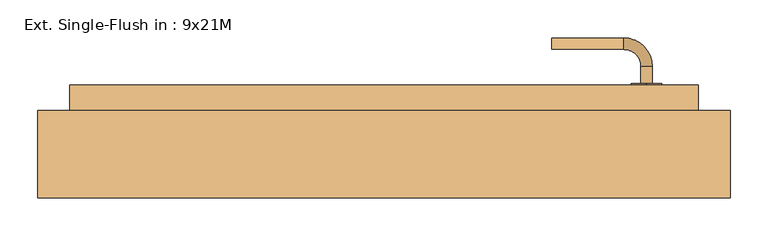
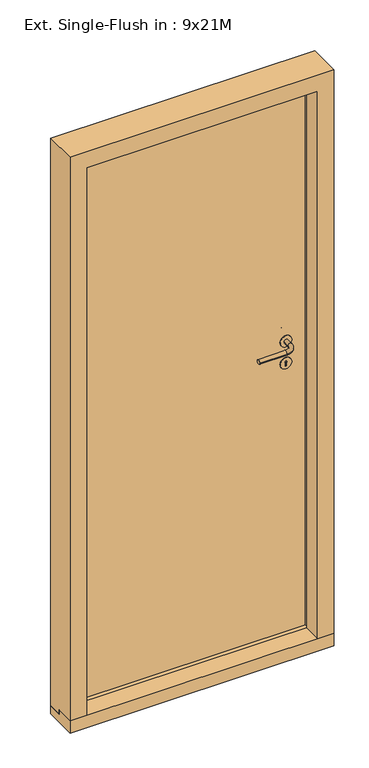
"""IFC4 building model written with IfcOpenShell, lengths in millimetres: door geometry, Ext. Single-Flush in : 9x21M."""

import ifcopenshell
import ifcopenshell.guid

model = None  # the IFC model being written
_history = None  # IfcOwnerHistory: only IFC2X3 demands one
_inside = {}  # id of a spatial element -> (the spatial element, [elements in it])
_under = {}  # id of a project, library or spatial element -> (it, [spatial elements below it])
_declared = {}  # id of a project -> (the project, [libraries it declares])
_typed = {}  # id of a type object -> (the type object, [elements of that type])
_made_of = {}  # id of a material, layer set ... -> (it, [elements and type objects made of it])


def new_model(schema):
    """Start an empty IFC model of exactly this schema.

    Asked for "IFC4X3", IfcOpenShell would pick the latest addendum, in which some entities
    have other attributes; the version numbers below select the first issue.
    IFC2X3 requires an IfcOwnerHistory on every rooted entity: one is made here for all.
    """
    global model, _history
    if schema == "IFC4X3":
        model = ifcopenshell.file(schema_version=(4, 3, 0, 0))
    else:
        model = ifcopenshell.file(schema=schema)
    _inside.clear()
    _under.clear()
    _declared.clear()
    _typed.clear()
    _made_of.clear()
    _history = None
    if model.schema == "IFC2X3":
        org = make("IfcOrganization", Name="unknown")
        user = make(
            "IfcPersonAndOrganization",
            ThePerson=make("IfcPerson", FamilyName="unknown"),
            TheOrganization=org,
        )
        app = make(
            "IfcApplication",
            ApplicationDeveloper=org,
            Version="unknown",
            ApplicationFullName="unknown",
            ApplicationIdentifier="unknown",
        )
        _history = make(
            "IfcOwnerHistory",
            OwningUser=user,
            OwningApplication=app,
            ChangeAction="ADDED",
            CreationDate=0,
        )
    return model


def make(cls, **values):
    """One entity of the class cls with the attributes given. An attribute that is None is left unset."""
    return model.create_entity(
        cls, **{name: value for name, value in values.items() if value is not None}
    )


def rooted(cls, **values):
    """An entity with a GlobalId (a new one), such as an element, a storey or a relation."""
    return make(cls, GlobalId=ifcopenshell.guid.new(), OwnerHistory=_history, **values)


def si_unit(unit_type, name, prefix=None):
    """IfcSIUnit, for example si_unit("LENGTHUNIT", "METRE", prefix="MILLI")."""
    return make("IfcSIUnit", UnitType=unit_type, Prefix=prefix, Name=name)


def assignment(units):
    """IfcUnitAssignment: the units of a project."""
    return None if units is None else make("IfcUnitAssignment", Units=units)


def point(xyz):
    """IfcCartesianPoint."""
    return None if xyz is None else make("IfcCartesianPoint", Coordinates=xyz)


def direction(xyz):
    """IfcDirection."""
    return None if xyz is None else make("IfcDirection", DirectionRatios=xyz)


def frame(location, z_axis=None, x_axis=None):
    """IfcAxis2Placement3D, a coordinate frame: its origin and axes. An axis left out is left unset."""
    return make(
        "IfcAxis2Placement3D",
        Location=point(location),
        Axis=direction(z_axis),
        RefDirection=direction(x_axis),
    )


def frame_2d(location, x_axis=None):
    """IfcAxis2Placement2D, a coordinate frame in the plane: its origin and x axis."""
    return make(
        "IfcAxis2Placement2D", Location=point(location), RefDirection=direction(x_axis)
    )


def origin():
    """The frame at (0, 0, 0) with its axes left unset."""
    return frame((0.0, 0.0, 0.0))


def place(relative_to, where):
    """IfcLocalPlacement: puts the frame where relative to a parent placement (None: the world)."""
    return make(
        "IfcLocalPlacement", PlacementRelTo=relative_to, RelativePlacement=where
    )


def context(
    kind, dimensions, precision=None, world=None, true_north=None, identifier=None
):
    """IfcGeometricRepresentationContext, for example the 3D "Model" context."""
    return make(
        "IfcGeometricRepresentationContext",
        ContextIdentifier=identifier,
        ContextType=kind,
        CoordinateSpaceDimension=dimensions,
        Precision=precision,
        WorldCoordinateSystem=world,
        TrueNorth=true_north,
    )


def project(units=None, contexts=None):
    """IfcProject with its units and contexts."""
    return rooted(
        "IfcProject",
        Name="project",
        RepresentationContexts=contexts,
        UnitsInContext=assignment(units),
    )


def spatial(cls, under=None, at=None, **own):
    """A site, building, storey or space (cls), placed at a placement, below another one or the project."""
    s = rooted(cls, ObjectPlacement=at, **own)
    if under is not None:
        _under.setdefault(under.id(), (under, []))[1].append(s)
    return s


def polyline(points):
    """IfcPolyline through the points."""
    return make("IfcPolyline", Points=[point(p) for p in points])


def circle_curve(where, radius):
    """IfcCircle in the frame where."""
    return make("IfcCircle", Position=where, Radius=radius)


def ellipse_curve(where, semi_axis1, semi_axis2):
    """IfcEllipse in the frame where."""
    return make(
        "IfcEllipse", Position=where, SemiAxis1=semi_axis1, SemiAxis2=semi_axis2
    )


def trimmed(basis, trim1, trim2, sense, master):
    """IfcTrimmedCurve: the piece of a basis curve between two trims."""
    return make(
        "IfcTrimmedCurve",
        BasisCurve=basis,
        Trim1=trim1,
        Trim2=trim2,
        SenseAgreement=sense,
        MasterRepresentation=master,
    )


def segment(curve, same_sense, transition):
    """IfcCompositeCurveSegment."""
    return make(
        "IfcCompositeCurveSegment",
        Transition=transition,
        SameSense=same_sense,
        ParentCurve=curve,
    )


def composite_curve(segments, self_intersect=None):
    """IfcCompositeCurve: segments joined end to end."""
    return make("IfcCompositeCurve", Segments=segments, SelfIntersect=self_intersect)


def outline(outer, holes=None, kind="AREA"):
    """IfcArbitraryClosedProfileDef: a profile drawn as a closed curve; with holes, ...WithVoids."""
    if holes is None:
        return make("IfcArbitraryClosedProfileDef", ProfileType=kind, OuterCurve=outer)
    return make(
        "IfcArbitraryProfileDefWithVoids",
        ProfileType=kind,
        OuterCurve=outer,
        InnerCurves=holes,
    )


def extrude(swept, where, along, depth):
    """IfcExtrudedAreaSolid: the profile swept, set in the frame where, extruded along a direction by depth."""
    return make(
        "IfcExtrudedAreaSolid",
        SweptArea=swept,
        Position=where,
        ExtrudedDirection=direction(along),
        Depth=depth,
    )


def faces_of(points, faces, orient=None, outer=None):
    """IfcFace entities. A face is a list of loops; a loop is a list of indices into points, from 0.

    orient and outer hold one flag for each loop. By default every Orientation is true, the
    first loop of a face is its IfcFaceOuterBound and the others are IfcFaceBound.
    """
    made = []
    for i, loops in enumerate(faces):
        bounds = []
        for j, loop in enumerate(loops):
            is_outer = j == 0 if outer is None else outer[i][j]
            bounds.append(
                make(
                    "IfcFaceOuterBound" if is_outer else "IfcFaceBound",
                    Bound=make("IfcPolyLoop", Polygon=[points[k] for k in loop]),
                    Orientation=True if orient is None else orient[i][j],
                )
            )
        made.append(make("IfcFace", Bounds=bounds))
    return made


def faceted_brep(points, faces, orient=None, outer=None, voids=None):
    """IfcFacetedBrep: a solid bounded by flat faces; with voids (closed shells), ...WithVoids."""
    shared = [point(p) for p in points]
    hull = make("IfcClosedShell", CfsFaces=faces_of(shared, faces, orient, outer))
    if voids is None:
        return make("IfcFacetedBrep", Outer=hull)
    return make(
        "IfcFacetedBrepWithVoids",
        Outer=hull,
        Voids=[
            make(cls, CfsFaces=faces_of(shared, fs, o, b)) for cls, fs, o, b in voids
        ],
    )


def shape(context_of_items, identifier, shape_type, items):
    """IfcShapeRepresentation: the items that make up one representation, for example the "Body"."""
    return make(
        "IfcShapeRepresentation",
        ContextOfItems=context_of_items,
        RepresentationIdentifier=identifier,
        RepresentationType=shape_type,
        Items=items,
    )


def source(mapping_origin, context_of_items, identifier, shape_type, items):
    """IfcRepresentationMap: a shape defined once, which mapped items show again and again."""
    return make(
        "IfcRepresentationMap",
        MappingOrigin=mapping_origin,
        MappedRepresentation=shape(context_of_items, identifier, shape_type, items),
    )


def transform(
    local_origin,
    x_axis=None,
    y_axis=None,
    z_axis=None,
    scale=None,
    scale2=None,
    scale3=None,
    uniform=True,
):
    """IfcCartesianTransformationOperator3D, or its non-uniform kind. x_axis, y_axis, z_axis: its Axis1, 2, 3."""
    if uniform:
        return make(
            "IfcCartesianTransformationOperator3D",
            Axis1=direction(x_axis),
            Axis2=direction(y_axis),
            LocalOrigin=point(local_origin),
            Scale=scale,
            Axis3=direction(z_axis),
        )
    return make(
        "IfcCartesianTransformationOperator3DnonUniform",
        Axis1=direction(x_axis),
        Axis2=direction(y_axis),
        LocalOrigin=point(local_origin),
        Scale=scale,
        Axis3=direction(z_axis),
        Scale2=scale2,
        Scale3=scale3,
    )


def mapped(mapping_source, mapping_target):
    """IfcMappedItem: shows the shape of a source again, moved by a transform."""
    return make(
        "IfcMappedItem", MappingSource=mapping_source, MappingTarget=mapping_target
    )


def made_of(thing, what):
    """Note that an element or type object is made of a material, layer set ...; save() writes the relation."""
    if what is not None:
        _made_of.setdefault(what.id(), (what, []))[1].append(thing)
    return thing


def element(
    cls,
    number,
    at=None,
    inside=None,
    cuts=None,
    type_object=None,
    material=None,
    context=None,
    identifier="Body",
    shape_type=None,
    held_by="IfcProductDefinitionShape",
    body=None,
    shapes=None,
    **own,
):
    """One element of the class cls, such as IfcWall. Its Tag is "e" and its number.

    at: its placement. inside: the storey or other place that contains it. cuts: it is an
    opening in that element (IfcRelVoidsElement). A single representation is given by context,
    identifier, shape_type and body (its items); several are given by shapes. held_by: the class
    of the entity that holds the representations. save() writes the other relations.
    """
    e = rooted(cls, Tag="e%d" % number, ObjectPlacement=at, **own)
    if body is not None:
        shapes = [shape(context, identifier, shape_type, body)]
    if shapes is not None:
        e.Representation = make(held_by, Representations=shapes)
    if inside is not None:
        _inside.setdefault(inside.id(), (inside, []))[1].append(e)
    if cuts is not None:
        rooted(
            "IfcRelVoidsElement", RelatingBuildingElement=cuts, RelatedOpeningElement=e
        )
    if type_object is not None:
        _typed.setdefault(type_object.id(), (type_object, []))[1].append(e)
    return made_of(e, material)


def aggregate(whole, parts):
    """IfcRelAggregates: a whole, such as a stair, and the parts it consists of."""
    return rooted("IfcRelAggregates", RelatingObject=whole, RelatedObjects=parts)


def save(model, path):
    """Write the relations noted so far, then the file.

    IfcRelAggregates (storeys below a building ...), IfcRelContainedInSpatialStructure (elements
    in a storey), IfcRelDefinesByType, IfcRelAssociatesMaterial and IfcRelDeclares: one each for
    every whole, place, type object, material and project.
    """
    for whole, parts in _under.values():
        aggregate(whole, parts)
    for where, things in _inside.values():
        rooted(
            "IfcRelContainedInSpatialStructure",
            RelatedElements=things,
            RelatingStructure=where,
        )
    for kind, things in _typed.values():
        rooted("IfcRelDefinesByType", RelatedObjects=things, RelatingType=kind)
    for what, things in _made_of.values():
        rooted("IfcRelAssociatesMaterial", RelatedObjects=things, RelatingMaterial=what)
    for by, libraries in _declared.values():
        rooted("IfcRelDeclares", RelatingContext=by, RelatedDefinitions=libraries)
    model.write(path)


def plane_surface(at):
    """IfcPlane: the flat surface through the origin of the frame at, square to its z axis."""
    return make("IfcPlane", Position=at)


def cylinder_surface(at, radius):
    """IfcCylindricalSurface: all points at the distance radius from the z axis of the frame at."""
    return make("IfcCylindricalSurface", Position=at, Radius=radius)


def revolved_surface(curve, axis_point, axis_direction):
    """IfcSurfaceOfRevolution: the curve turned about the line through axis_point along axis_direction."""
    return make(
        "IfcSurfaceOfRevolution",
        SweptCurve=make("IfcArbitraryOpenProfileDef", ProfileType="CURVE", Curve=curve),
        AxisPosition=make("IfcAxis1Placement", Location=point(axis_point), Axis=direction(axis_direction)),
    )


def advanced_brep(points, edges, surfaces, faces):
    """IfcAdvancedBrep: a solid bounded by faces that lie on surfaces and meet in shared edges.

    An edge is (start, end): straight between two places in points (the first is 0);
    or (start, end, curve); or (start, end, curve, False) where it runs against its curve.
    A face is (place in surfaces, loops), or (place, loops, False) where it looks against
    its surface's normal. A loop lists edges by number (the first is 1), with a minus sign
    where the edge is run from its end to its start. The first loop is the outer one.
    """
    corners = [point(p) for p in points]
    vertices = [make("IfcVertexPoint", VertexGeometry=c) for c in corners]
    made = []
    for start, end, *more in edges:
        made.append(
            make(
                "IfcEdgeCurve",
                EdgeStart=vertices[start],
                EdgeEnd=vertices[end],
                EdgeGeometry=more[0] if more else make("IfcPolyline", Points=[corners[start], corners[end]]),
                SameSense=more[1] if len(more) > 1 else True,
            )
        )
    hull = []
    for where, loops, *sense in faces:
        bounds = []
        for j, loop in enumerate(loops):
            ring = [make("IfcOrientedEdge", EdgeElement=made[abs(k) - 1], Orientation=k > 0) for k in loop]
            bounds.append(
                make(
                    "IfcFaceOuterBound" if j == 0 else "IfcFaceBound",
                    Bound=make("IfcEdgeLoop", EdgeList=ring),
                    Orientation=True,
                )
            )
        hull.append(make("IfcAdvancedFace", Bounds=bounds, FaceSurface=surfaces[where], SameSense=sense[0] if sense else True))
    return make("IfcAdvancedBrep", Outer=make("IfcClosedShell", CfsFaces=hull))


def ext_single_flush_in_9x21m_f1e34a21(model_context):
    return source(origin(), model_context, "Body", "SolidModel", [
        extrude(outline(composite_curve([segment(trimmed(circle_curve(frame_2d((1090.0, 346.0)), 20.0), [point((1070.0, 346.0))], [point((1110.0, 346.0))], False, "CARTESIAN"), True, "CONTINUOUS"), segment(trimmed(circle_curve(frame_2d((1090.0, 346.0)), 20.0), [point((1110.0, 346.0))], [point((1070.0, 346.0))], False, "CARTESIAN"), True, "CONTINUOUS")], self_intersect=False)), frame((0.0, -35.0, 0.0), z_axis=(0.0, 1.0, 0.0), x_axis=(0.0, 0.0, 1.0)), (0.0, 0.0, 1.0), 2.0),
        advanced_brep(
        [(353.5, -33.0, 1090.0), (338.5, -33.0, 1090.0), (338.5, -10.5, 1090.0), (353.5, -10.5, 1090.0), (316.0, 12.0, 1090.0), (316.0, 27.0, 1090.0), (221.0, 12.0, 1090.0), (221.0, 27.0, 1090.0)],
        [
            (0, 1, circle_curve(frame((346.0, -33.0, 1090.0), z_axis=(0.0, -1.0, 0.0), x_axis=(-1.0, 0.0, 0.0)), 7.5)),
            (1, 0, circle_curve(frame((346.0, -33.0, 1090.0), z_axis=(0.0, -1.0, 0.0), x_axis=(-1.0, 0.0, 0.0)), 7.5)),
            (1, 2),
            (2, 3, circle_curve(frame((346.0, -10.5, 1090.0), z_axis=(0.0, -1.0, 0.0), x_axis=(-1.0, 0.0, 0.0)), 7.5)),
            (3, 0),
            (3, 2, circle_curve(frame((346.0, -10.5, 1090.0), z_axis=(0.0, -1.0, 0.0), x_axis=(-1.0, 0.0, 0.0)), 7.5)),
            (4, 5, circle_curve(frame((316.0, 19.5, 1090.0), z_axis=(1.0, 0.0, 0.0), x_axis=(0.0, -1.0, 0.0)), 7.5)),
            (5, 3, circle_curve(frame((316.0, -10.5, 1090.0), z_axis=(0.0, 0.0, -1.0), x_axis=(1.0, 0.0, 0.0)), 37.5)),
            (2, 4, circle_curve(frame((316.0, -10.5, 1090.0), z_axis=(0.0, 0.0, 1.0), x_axis=(1.0, 0.0, 0.0)), 22.5)),
            (5, 4, circle_curve(frame((316.0, 19.5, 1090.0), z_axis=(1.0, 0.0, 0.0), x_axis=(0.0, -1.0, 0.0)), 7.5)),
            (4, 6),
            (6, 7, circle_curve(frame((221.0, 19.5, 1090.0), z_axis=(1.0, 0.0, 0.0), x_axis=(0.0, -1.0, 0.0)), 7.5)),
            (7, 5),
            (7, 6, circle_curve(frame((221.0, 19.5, 1090.0), z_axis=(1.0, 0.0, 0.0), x_axis=(0.0, -1.0, 0.0)), 7.5)),
        ],
        [
            plane_surface(frame((346.0, -33.0, 1090.0), z_axis=(0.0, -1.0, 0.0), x_axis=(0.0, 0.0, -1.0))),
            cylinder_surface(frame((346.0, -33.0, 1090.0), z_axis=(0.0, -1.0, 0.0), x_axis=(-1.0, 0.0, 0.0)), 7.5),
            revolved_surface(trimmed(ellipse_curve(frame((346.0, -10.5, 1090.0), z_axis=(0.0, 1.0, 0.0), x_axis=(-1.0, 0.0, 0.0)), 7.5, 7.5), [point((353.5, -10.5, 1090.0))], [point((338.5, -10.5, 1090.0))], True, "CARTESIAN"), (316.0, -10.5, 1090.0), (0.0, 0.0, -1.0)),
            revolved_surface(trimmed(ellipse_curve(frame((346.0, -10.5, 1090.0), z_axis=(0.0, 1.0, 0.0), x_axis=(-1.0, 0.0, 0.0)), 7.5, 7.5), [point((338.5, -10.5, 1090.0))], [point((353.5, -10.5, 1090.0))], True, "CARTESIAN"), (316.0, -10.5, 1090.0), (0.0, 0.0, -1.0)),
            cylinder_surface(frame((316.0, 19.5, 1090.0), z_axis=(1.0, 0.0, 0.0), x_axis=(0.0, -1.0, 0.0)), 7.5),
            plane_surface(frame((221.0, 19.5, 1090.0), z_axis=(-1.0, 0.0, 0.0), x_axis=(0.0, 0.0, -1.0))),
        ],
        [
            (0, [[1, 2]]),
            (1, [[3, 4, 5, -2]]),
            (1, [[-5, 6, -3, -1]]),
            (2, [[7, 8, -4, 9]]),
            (3, [[10, -9, -6, -8]]),
            (4, [[11, 12, 13, -7]]),
            (4, [[-13, 14, -11, -10]]),
            (5, [[-12, -14]]),
        ],
    ),
        extrude(outline(composite_curve([segment(trimmed(circle_curve(frame_2d((1010.0, 346.0)), 20.0), [point((990.0, 346.0))], [point((1030.0, 346.0))], False, "CARTESIAN"), True, "CONTINUOUS"), segment(trimmed(circle_curve(frame_2d((1010.0, 346.0)), 20.0), [point((1030.0, 346.0))], [point((990.0, 346.0))], False, "CARTESIAN"), True, "CONTINUOUS")], self_intersect=False), holes=[composite_curve([segment(polyline([(1012.4019238, 347.5), (1000.0, 347.5), (1000.0, 344.5), (1012.4019238, 344.5)]), True, "CONTINUOUS"), segment(trimmed(circle_curve(frame_2d((1015.0, 346.0)), 3.0), [point((1012.4019238, 344.5))], [point((1012.4019238, 347.5))], True, "CARTESIAN"), True, "CONTINUOUS")], self_intersect=False)]), frame((0.0, -35.0, 0.0), z_axis=(0.0, 1.0, 0.0), x_axis=(0.0, 0.0, 1.0)), (0.0, 0.0, 1.0), 2.0),
        extrude(outline(composite_curve([segment(trimmed(circle_curve(frame_2d((1090.0, 346.0)), 20.0), [point((1070.0, 346.0))], [point((1110.0, 346.0))], False, "CARTESIAN"), True, "CONTINUOUS"), segment(trimmed(circle_curve(frame_2d((1090.0, 346.0)), 20.0), [point((1110.0, 346.0))], [point((1070.0, 346.0))], False, "CARTESIAN"), True, "CONTINUOUS")], self_intersect=False)), frame((0.0, -87.0, 0.0), z_axis=(0.0, 1.0, 0.0), x_axis=(0.0, 0.0, 1.0)), (0.0, 0.0, 1.0), 2.0),
        advanced_brep(
        [(353.5, -87.0, 1090.0), (338.5, -87.0, 1090.0), (353.5, -109.5, 1090.0), (338.5, -109.5, 1090.0), (316.0, -132.0, 1090.0), (316.0, -147.0, 1090.0), (221.0, -147.0, 1090.0), (221.0, -132.0, 1090.0)],
        [
            (0, 1, circle_curve(frame((346.0, -87.0, 1090.0), z_axis=(0.0, 1.0, 0.0), x_axis=(-1.0, 0.0, 0.0)), 7.5)),
            (1, 0, circle_curve(frame((346.0, -87.0, 1090.0), z_axis=(0.0, 1.0, 0.0), x_axis=(-1.0, 0.0, 0.0)), 7.5)),
            (0, 2),
            (2, 3, circle_curve(frame((346.0, -109.5, 1090.0), z_axis=(0.0, 1.0, 0.0), x_axis=(-1.0, 0.0, 0.0)), 7.5)),
            (3, 1),
            (3, 2, circle_curve(frame((346.0, -109.5, 1090.0), z_axis=(0.0, 1.0, 0.0), x_axis=(-1.0, 0.0, 0.0)), 7.5)),
            (4, 3, circle_curve(frame((316.0, -109.5, 1090.0), z_axis=(0.0, 0.0, 1.0), x_axis=(1.0, 0.0, 0.0)), 22.5)),
            (2, 5, circle_curve(frame((316.0, -109.5, 1090.0), z_axis=(0.0, 0.0, -1.0), x_axis=(1.0, 0.0, 0.0)), 37.5)),
            (5, 4, circle_curve(frame((316.0, -139.5, 1090.0), z_axis=(1.0, 0.0, 0.0), x_axis=(0.0, 1.0, 0.0)), 7.5)),
            (4, 5, circle_curve(frame((316.0, -139.5, 1090.0), z_axis=(1.0, 0.0, 0.0), x_axis=(0.0, 1.0, 0.0)), 7.5)),
            (5, 6),
            (6, 7, circle_curve(frame((221.0, -139.5, 1090.0), z_axis=(1.0, 0.0, 0.0), x_axis=(0.0, 1.0, 0.0)), 7.5)),
            (7, 4),
            (7, 6, circle_curve(frame((221.0, -139.5, 1090.0), z_axis=(1.0, 0.0, 0.0), x_axis=(0.0, 1.0, 0.0)), 7.5)),
        ],
        [
            plane_surface(frame((346.0, -87.0, 1090.0), z_axis=(0.0, 1.0, 0.0), x_axis=(0.0, 0.0, -1.0))),
            cylinder_surface(frame((346.0, -87.0, 1090.0), z_axis=(0.0, 1.0, 0.0), x_axis=(-1.0, 0.0, 0.0)), 7.5),
            revolved_surface(trimmed(ellipse_curve(frame((346.0, -109.5, 1090.0), z_axis=(0.0, 1.0, 0.0), x_axis=(-1.0, 0.0, 0.0)), 7.5, 7.5), [point((353.5, -109.5, 1090.0))], [point((338.5, -109.5, 1090.0))], True, "CARTESIAN"), (316.0, -109.5, 1090.0), (0.0, 0.0, -1.0)),
            revolved_surface(trimmed(ellipse_curve(frame((346.0, -109.5, 1090.0), z_axis=(0.0, 1.0, 0.0), x_axis=(-1.0, 0.0, 0.0)), 7.5, 7.5), [point((338.5, -109.5, 1090.0))], [point((353.5, -109.5, 1090.0))], True, "CARTESIAN"), (316.0, -109.5, 1090.0), (0.0, 0.0, -1.0)),
            cylinder_surface(frame((316.0, -139.5, 1090.0), z_axis=(1.0, 0.0, 0.0), x_axis=(0.0, 1.0, 0.0)), 7.5),
            plane_surface(frame((221.0, -139.5, 1090.0), z_axis=(-1.0, 0.0, 0.0), x_axis=(0.0, 0.0, -1.0))),
        ],
        [
            (0, [[1, 2]]),
            (1, [[-1, 3, 4, 5]]),
            (1, [[-2, -5, 6, -3]]),
            (2, [[7, -4, 8, 9]]),
            (3, [[-8, -6, -7, 10]]),
            (4, [[-9, 11, 12, 13]]),
            (4, [[-10, -13, 14, -11]]),
            (5, [[-14, -12]]),
        ],
    ),
        extrude(outline(composite_curve([segment(trimmed(circle_curve(frame_2d((1010.0, 346.0)), 20.0), [point((990.0, 346.0))], [point((1030.0, 346.0))], False, "CARTESIAN"), True, "CONTINUOUS"), segment(trimmed(circle_curve(frame_2d((1010.0, 346.0)), 20.0), [point((1030.0, 346.0))], [point((990.0, 346.0))], False, "CARTESIAN"), True, "CONTINUOUS")], self_intersect=False), holes=[composite_curve([segment(polyline([(1012.4019238, 347.5), (1000.0, 347.5), (1000.0, 344.5), (1012.4019238, 344.5)]), True, "CONTINUOUS"), segment(trimmed(circle_curve(frame_2d((1015.0, 346.0)), 3.0), [point((1012.4019238, 344.5))], [point((1012.4019238, 347.5))], True, "CARTESIAN"), True, "CONTINUOUS")], self_intersect=False)]), frame((0.0, -87.0, 0.0), z_axis=(0.0, 1.0, 0.0), x_axis=(0.0, 0.0, 1.0)), (0.0, 0.0, 1.0), 2.0),
        faceted_brep([(-414.0, -69.0, 2058.0), (-414.0, -69.0, 30.0), (-456.0, -69.0, 30.0), (-456.0, -69.0, 2100.0), (456.0, -69.0, 2100.0), (456.0, -69.0, 30.0), (414.0, -69.0, 30.0), (414.0, -69.0, 2058.0), (414.0, -119.0, 30.0), (414.0, -119.0, 45.0), (414.0, -119.0, 2058.0), (456.0, -119.0, 30.0), (-456.0, -119.0, 30.0), (-414.0, -119.0, 30.0), (456.0, -184.0, 2100.0), (456.0, -184.0, 45.0), (456.0, -119.0, 45.0), (-456.0, -119.0, 45.0), (-456.0, -184.0, 45.0), (-456.0, -184.0, 2100.0), (-414.0, -119.0, 2058.0), (-414.0, -119.0, 45.0), (-399.0, -184.0, 45.0), (-399.0, -184.0, 2043.0), (399.0, -184.0, 2043.0), (399.0, -184.0, 45.0), (399.0, -119.0, 45.0), (-399.0, -119.0, 45.0), (399.0, -119.0, 2043.0), (-399.0, -119.0, 2043.0)], [[[0, 1, 2, 3, 4, 5, 6, 7]], [[7, 6, 8, 9, 10]], [[8, 6, 5, 11]], [[12, 2, 1, 13]], [[14, 15, 16, 11, 5, 4]], [[3, 2, 12, 17, 18, 19]], [[20, 21, 13, 1, 0]], [[19, 18, 22, 23, 24, 25, 15, 14]], [[16, 15, 25, 26, 9]], [[21, 27, 22, 18, 17]], [[11, 16, 9, 8]], [[13, 21, 17, 12]], [[28, 26, 25, 24]], [[23, 22, 27, 29]], [[29, 27, 21, 20, 10, 9, 26, 28]], [[3, 19, 14, 4]], [[23, 29, 28, 24]], [[7, 10, 20, 0]]]),
        extrude(outline(polyline([(-414.0, -85.0), (-414.0, -35.0), (414.0, -35.0), (414.0, -85.0), (-414.0, -85.0)])), frame((0.0, 0.0, 30.0), z_axis=(0.0, 0.0, 1.0), x_axis=(1.0, 0.0, 0.0)), (0.0, 0.0, 1.0), 2028.0),
        extrude(outline(polyline([(-69.0, 30.0), (-69.0, 0.0), (-184.0, 0.0), (-184.0, 45.0), (-119.0, 45.0), (-119.0, 30.0), (-69.0, 30.0)])), frame((-456.0, 0.0, 0.0), z_axis=(1.0, 0.0, 0.0), x_axis=(0.0, 1.0, 0.0)), (0.0, 0.0, 1.0), 912.0),
    ])


if __name__ == "__main__":
    model = new_model("IFC4")
    model_context = context("Model", 3, world=origin())
    ifc_project = project(units=[si_unit("LENGTHUNIT", "METRE", prefix="MILLI")], contexts=[model_context])
    site = spatial("IfcSite", under=ifc_project)
    building = spatial("IfcBuilding", under=site)
    placement = place(None, origin())
    ext_single_flush_in_9x21m_shape = ext_single_flush_in_9x21m_f1e34a21(model_context)
    element("IfcDoor", 1, ObjectType="Ext. Single-Flush in : 9x21M", at=placement, inside=building, context=model_context, shape_type="MappedRepresentation", body=[
        mapped(ext_single_flush_in_9x21m_shape, transform((0.0, 0.0, 0.0), x_axis=(1.0, 0.0, 0.0), y_axis=(0.0, 1.0, 0.0), z_axis=(0.0, 0.0, 1.0))),
    ])
    save(model, "model.ifc")

# Revit data of these elements
# Type "Ext. Single-Flush in : 9x21M"
#   Type Mark = "62"
#   Sound Rating = ""
#   Opening Side [instance default] = "in"
#   Hinge Side [instance default] = ""
#   Creator Build [instance default] = "2017.0301.0"
#   Creator Organization [instance default] = "© Danish Educational Content"
#   Creator Name [instance default] = "© Erik Falck Jørgensen"
#   Analytic Construction = "<None>"
#   length#5 = 912 mm
#   length#4 = 120 mm
#   length#3 = 30 mm
#   length#2 = 57 mm
#   length#1 = 0 mm
#   Thickness = 50 mm
#   Seal Width = 12 mm
#   Rough Width = 912 mm
#   Rough Height = 2100 mm
#   Rebate Depth = 50 mm
#   Rabbet Width = 15 mm
#   Rabbet Depth = 50 mm
#   Height = 2088 mm
#   Width = 888 mm
#   Handle From Side = 110 mm
#   Handle From Bottom = 1090 mm
#   Exterior Direction [instance default] = 0.00°
#   Case Depth = 115 mm
#   Case Width = 45 mm
#   Threshold = yes
#   Sealing = no
#   Hinging = yes
#   Wall Closure = 1
#   Function = 1
#   Panel = none
#   Handle Finish = none
#   Handle = element 628255
#   Case/Transom = none
#   Assembly Code = ""
# Element 1 (IfcDoor, "Ext. Single-Flush in : 9x21M")
#   Materials on its faces: "Stainless Steel, Polished", "Default Frame/Mullion (Interior/Exterior)", "Default Door Panel (Exterior/Interior)"
# Materials
#   "Stainless Steel, Polished": class "Metal", colour RGB 180 180 180, transparency 0, Description = "Rustfri stål, poleret", Cost = 0
#   "Default Frame/Mullion (Interior/Exterior)": class "Generic", colour RGB 205 205 205, transparency 0, Description = "Udefineret karm/ramme materiale", Cost = 0
#   "Default Door Panel (Exterior/Interior)": class "Generic", colour RGB 205 205 205, transparency 0, Description = "Udefineret dørplade materiale", Cost = 0
